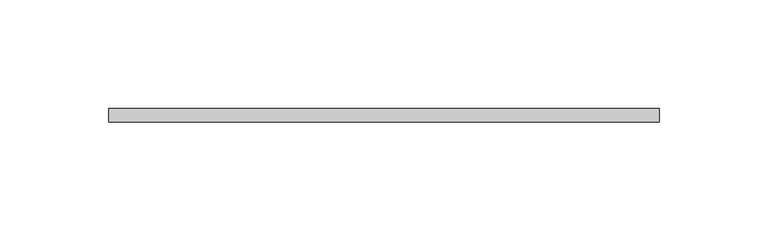
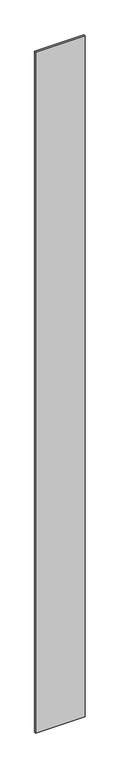
"""IFC4 building model written with IfcOpenShell, lengths in millimetres: proxy geometry, Inner panel1:Inner panel:306176:Inner panel:306176 : Inner panel1:Inner panel:306176:300391:Inner panel:306176:Inner panel:306176 : Inner panel1:Inner panel:306176:300391 : Inner panel1:Inner panel:306176:Inner panel:306176 : Inner panel1:Inner panel:306176:300391:5 : Inner panel1:Inner panel:306176:Inner panel:306176 : Inner panel1:Inner panel:306176:300391:Inner panel:306176:Inner panel:306176 : Inner panel1:Inner panel:306176:300391 : Inner panel1:Inner panel:306176:Inner panel:306176 : Inner panel1:Inner panel:306176:300391:300168."""

from ifc_helpers import new_model, si_unit, frame, origin, place, context, project, spatial, polyline, outline, extrude, source, transform, mapped, element, save


def generic_models_26e58b4d(model_context):
    return source(origin(), model_context, "Body", "SweptSolid", [
        extrude(outline(polyline([(595956.0015778, -578778.4413841), (595956.0015778, -578772.0913841), (596209.6582416, -578772.0913841), (596209.6582416, -578778.4413841), (595956.0015778, -578778.4413841)])), frame((0.0, 0.0, 25.4), z_axis=(0.0, 0.0, 1.0), x_axis=(1.0, 0.0, 0.0)), (0.0, 0.0, 1.0), 3689.35),
    ])


if __name__ == "__main__":
    model = new_model("IFC4")
    model_context = context("Model", 3, world=origin())
    ifc_project = project(units=[si_unit("LENGTHUNIT", "METRE", prefix="MILLI")], contexts=[model_context])
    site = spatial("IfcSite", under=ifc_project)
    building = spatial("IfcBuilding", under=site)
    placement = place(None, origin())
    generic_models_shape = generic_models_26e58b4d(model_context)
    element("IfcBuildingElementProxy", 1, Name="Inner panel1:Inner panel:306176:Inner panel:306176 : Inner panel1:Inner panel:306176:300391:Inner panel:306176:Inner panel:306176 : Inner panel1:Inner panel:306176:300391 : Inner panel1:Inner panel:306176:Inner panel:306176 : Inner panel1:Inner panel:306176:300391:5 : Inner panel1:Inner panel:306176:Inner panel:306176 : Inner panel1:Inner panel:306176:300391:Inner panel:306176:Inner panel:306176 : Inner panel1:Inner panel:306176:300391 : Inner panel1:Inner panel:306176:Inner panel:306176 : Inner panel1:Inner panel:306176:300391:300168", ObjectType="Inner panel1:Inner panel:306176:Inner panel:306176 : Inner panel1:Inner panel:306176:300391:Inner panel:306176:Inner panel:306176 : Inner panel1:Inner panel:306176:300391 : Inner panel1:Inner panel:306176:Inner panel:306176 : Inner panel1:Inner panel:306176:300391:5 : Inner panel1:Inner panel:306176:Inner panel:306176 : Inner panel1:Inner panel:306176:300391:Inner panel:306176:Inner panel:306176 : Inner panel1:Inner panel:306176:300391 : Inner panel1:Inner panel:306176:Inner panel:306176 : Inner panel1:Inner panel:306176:300391:300168", at=placement, inside=building, context=model_context, shape_type="MappedRepresentation", body=[
        mapped(generic_models_shape, transform((0.0, 0.0, 0.0), x_axis=(1.0, 0.0, 0.0), y_axis=(0.0, 1.0, 0.0), z_axis=(0.0, 0.0, 1.0))),
    ])
    save(model, "model.ifc")

# Revit data of these elements
# Type "Inner panel1:Inner panel:306176:Inner panel:306176 : Inner panel1:Inner panel:306176:300391:Inner panel:306176:Inner panel:306176 : Inner panel1:Inner panel:306176:300391 : Inner panel1:Inner panel:306176:Inner panel:306176 : Inner panel1:Inner panel:306176:300391:5 : Inner panel1:Inner panel:306176:Inner panel:306176 : Inner panel1:Inner panel:306176:300391:Inner panel:306176:Inner panel:306176 : Inner panel1:Inner panel:306176:300391 : Inner panel1:Inner panel:306176:Inner panel:306176 : Inner panel1:Inner panel:306176:300391:300168"
#   NameOverride = "Inner panel1:Inner panel:306176:Inner panel:306176 : Inner panel1:Inner panel:306176:300391:Inner panel:306176:Inner panel:306176 : Inner panel1:Inner panel:306176:300391 : Inner panel1:Inner panel:306176:Inner panel:306176 : Inner panel1:Inner panel:306176:300391:300168"
#   ObjectTypeOverride = "Inner panel:306176:Inner panel:306176 : Inner panel1:Inner panel:306176:300391 : Inner panel1:Inner panel:306176:Inner panel:306176 : Inner panel1:Inner panel:306176:300391"
#   Reference = "Inner panel"
#   Tag = "300168"
# Element 1 (IfcBuildingElementProxy, "Inner panel1:Inner panel:306176:Inner panel:306176 : Inner panel1:Inner panel:306176:300391:Inner panel:306176:Inner panel:306176 : Inner panel1:Inner panel:306176:300391 : Inner panel1:Inner panel:306176:Inner panel:306176 : Inner panel1:Inner panel:306176:300391:5 : Inner panel1:Inner panel:306176:Inner panel:306176 : Inner panel1:Inner panel:306176:300391:Inner panel:306176:Inner panel:306176 : Inner panel1:Inner panel:306176:300391 : Inner panel1:Inner panel:306176:Inner panel:306176 : Inner panel1:Inner panel:306176:300391:300168")
#   Materials on its faces: "1/4\" CEMENT BOARD"
# Materials
#   "1/4\" CEMENT BOARD": class "Generic", colour RGB 234 234 234, transparency 0, Cost = 0
